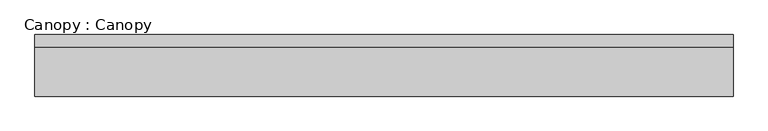
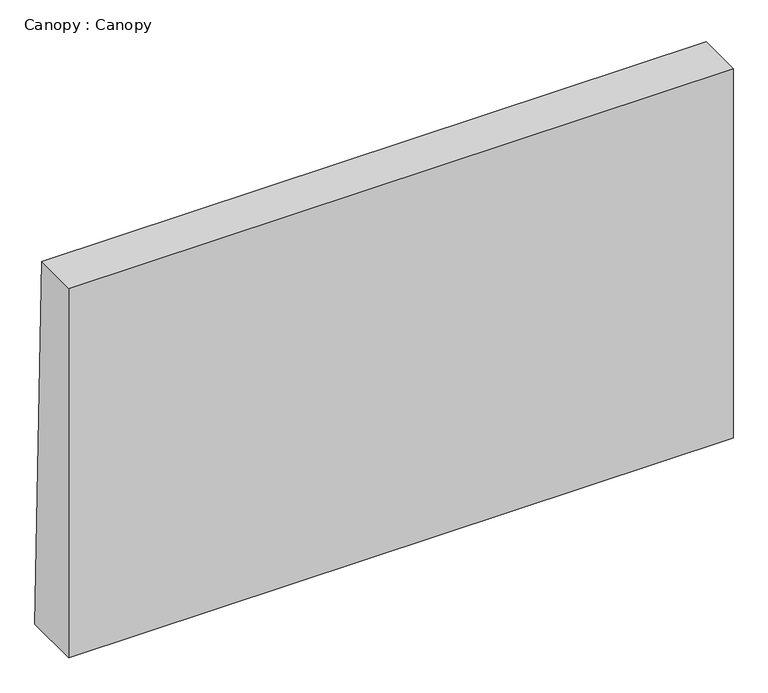
"""IFC4 building model written with IfcOpenShell, lengths in millimetres: proxy geometry, Canopy : Canopy."""

import ifcopenshell
import ifcopenshell.guid

model = None  # the IFC model being written
_history = None  # IfcOwnerHistory: only IFC2X3 demands one
_inside = {}  # id of a spatial element -> (the spatial element, [elements in it])
_under = {}  # id of a project, library or spatial element -> (it, [spatial elements below it])
_declared = {}  # id of a project -> (the project, [libraries it declares])
_typed = {}  # id of a type object -> (the type object, [elements of that type])
_made_of = {}  # id of a material, layer set ... -> (it, [elements and type objects made of it])


def new_model(schema):
    """Start an empty IFC model of exactly this schema.

    Asked for "IFC4X3", IfcOpenShell would pick the latest addendum, in which some entities
    have other attributes; the version numbers below select the first issue.
    IFC2X3 requires an IfcOwnerHistory on every rooted entity: one is made here for all.
    """
    global model, _history
    if schema == "IFC4X3":
        model = ifcopenshell.file(schema_version=(4, 3, 0, 0))
    else:
        model = ifcopenshell.file(schema=schema)
    _inside.clear()
    _under.clear()
    _declared.clear()
    _typed.clear()
    _made_of.clear()
    _history = None
    if model.schema == "IFC2X3":
        org = make("IfcOrganization", Name="unknown")
        user = make(
            "IfcPersonAndOrganization",
            ThePerson=make("IfcPerson", FamilyName="unknown"),
            TheOrganization=org,
        )
        app = make(
            "IfcApplication",
            ApplicationDeveloper=org,
            Version="unknown",
            ApplicationFullName="unknown",
            ApplicationIdentifier="unknown",
        )
        _history = make(
            "IfcOwnerHistory",
            OwningUser=user,
            OwningApplication=app,
            ChangeAction="ADDED",
            CreationDate=0,
        )
    return model


def make(cls, **values):
    """One entity of the class cls with the attributes given. An attribute that is None is left unset."""
    return model.create_entity(
        cls, **{name: value for name, value in values.items() if value is not None}
    )


def rooted(cls, **values):
    """An entity with a GlobalId (a new one), such as an element, a storey or a relation."""
    return make(cls, GlobalId=ifcopenshell.guid.new(), OwnerHistory=_history, **values)


def si_unit(unit_type, name, prefix=None):
    """IfcSIUnit, for example si_unit("LENGTHUNIT", "METRE", prefix="MILLI")."""
    return make("IfcSIUnit", UnitType=unit_type, Prefix=prefix, Name=name)


def assignment(units):
    """IfcUnitAssignment: the units of a project."""
    return None if units is None else make("IfcUnitAssignment", Units=units)


def point(xyz):
    """IfcCartesianPoint."""
    return None if xyz is None else make("IfcCartesianPoint", Coordinates=xyz)


def direction(xyz):
    """IfcDirection."""
    return None if xyz is None else make("IfcDirection", DirectionRatios=xyz)


def frame(location, z_axis=None, x_axis=None):
    """IfcAxis2Placement3D, a coordinate frame: its origin and axes. An axis left out is left unset."""
    return make(
        "IfcAxis2Placement3D",
        Location=point(location),
        Axis=direction(z_axis),
        RefDirection=direction(x_axis),
    )


def origin():
    """The frame at (0, 0, 0) with its axes left unset."""
    return frame((0.0, 0.0, 0.0))


def place(relative_to, where):
    """IfcLocalPlacement: puts the frame where relative to a parent placement (None: the world)."""
    return make(
        "IfcLocalPlacement", PlacementRelTo=relative_to, RelativePlacement=where
    )


def context(
    kind, dimensions, precision=None, world=None, true_north=None, identifier=None
):
    """IfcGeometricRepresentationContext, for example the 3D "Model" context."""
    return make(
        "IfcGeometricRepresentationContext",
        ContextIdentifier=identifier,
        ContextType=kind,
        CoordinateSpaceDimension=dimensions,
        Precision=precision,
        WorldCoordinateSystem=world,
        TrueNorth=true_north,
    )


def project(units=None, contexts=None):
    """IfcProject with its units and contexts."""
    return rooted(
        "IfcProject",
        Name="project",
        RepresentationContexts=contexts,
        UnitsInContext=assignment(units),
    )


def spatial(cls, under=None, at=None, **own):
    """A site, building, storey or space (cls), placed at a placement, below another one or the project."""
    s = rooted(cls, ObjectPlacement=at, **own)
    if under is not None:
        _under.setdefault(under.id(), (under, []))[1].append(s)
    return s


def polyline(points):
    """IfcPolyline through the points."""
    return make("IfcPolyline", Points=[point(p) for p in points])


def outline(outer, holes=None, kind="AREA"):
    """IfcArbitraryClosedProfileDef: a profile drawn as a closed curve; with holes, ...WithVoids."""
    if holes is None:
        return make("IfcArbitraryClosedProfileDef", ProfileType=kind, OuterCurve=outer)
    return make(
        "IfcArbitraryProfileDefWithVoids",
        ProfileType=kind,
        OuterCurve=outer,
        InnerCurves=holes,
    )


def extrude(swept, where, along, depth):
    """IfcExtrudedAreaSolid: the profile swept, set in the frame where, extruded along a direction by depth."""
    return make(
        "IfcExtrudedAreaSolid",
        SweptArea=swept,
        Position=where,
        ExtrudedDirection=direction(along),
        Depth=depth,
    )


def shape(context_of_items, identifier, shape_type, items):
    """IfcShapeRepresentation: the items that make up one representation, for example the "Body"."""
    return make(
        "IfcShapeRepresentation",
        ContextOfItems=context_of_items,
        RepresentationIdentifier=identifier,
        RepresentationType=shape_type,
        Items=items,
    )


def source(mapping_origin, context_of_items, identifier, shape_type, items):
    """IfcRepresentationMap: a shape defined once, which mapped items show again and again."""
    return make(
        "IfcRepresentationMap",
        MappingOrigin=mapping_origin,
        MappedRepresentation=shape(context_of_items, identifier, shape_type, items),
    )


def transform(
    local_origin,
    x_axis=None,
    y_axis=None,
    z_axis=None,
    scale=None,
    scale2=None,
    scale3=None,
    uniform=True,
):
    """IfcCartesianTransformationOperator3D, or its non-uniform kind. x_axis, y_axis, z_axis: its Axis1, 2, 3."""
    if uniform:
        return make(
            "IfcCartesianTransformationOperator3D",
            Axis1=direction(x_axis),
            Axis2=direction(y_axis),
            LocalOrigin=point(local_origin),
            Scale=scale,
            Axis3=direction(z_axis),
        )
    return make(
        "IfcCartesianTransformationOperator3DnonUniform",
        Axis1=direction(x_axis),
        Axis2=direction(y_axis),
        LocalOrigin=point(local_origin),
        Scale=scale,
        Axis3=direction(z_axis),
        Scale2=scale2,
        Scale3=scale3,
    )


def mapped(mapping_source, mapping_target):
    """IfcMappedItem: shows the shape of a source again, moved by a transform."""
    return make(
        "IfcMappedItem", MappingSource=mapping_source, MappingTarget=mapping_target
    )


def made_of(thing, what):
    """Note that an element or type object is made of a material, layer set ...; save() writes the relation."""
    if what is not None:
        _made_of.setdefault(what.id(), (what, []))[1].append(thing)
    return thing


def element(
    cls,
    number,
    at=None,
    inside=None,
    cuts=None,
    type_object=None,
    material=None,
    context=None,
    identifier="Body",
    shape_type=None,
    held_by="IfcProductDefinitionShape",
    body=None,
    shapes=None,
    **own,
):
    """One element of the class cls, such as IfcWall. Its Tag is "e" and its number.

    at: its placement. inside: the storey or other place that contains it. cuts: it is an
    opening in that element (IfcRelVoidsElement). A single representation is given by context,
    identifier, shape_type and body (its items); several are given by shapes. held_by: the class
    of the entity that holds the representations. save() writes the other relations.
    """
    e = rooted(cls, Tag="e%d" % number, ObjectPlacement=at, **own)
    if body is not None:
        shapes = [shape(context, identifier, shape_type, body)]
    if shapes is not None:
        e.Representation = make(held_by, Representations=shapes)
    if inside is not None:
        _inside.setdefault(inside.id(), (inside, []))[1].append(e)
    if cuts is not None:
        rooted(
            "IfcRelVoidsElement", RelatingBuildingElement=cuts, RelatedOpeningElement=e
        )
    if type_object is not None:
        _typed.setdefault(type_object.id(), (type_object, []))[1].append(e)
    return made_of(e, material)


def aggregate(whole, parts):
    """IfcRelAggregates: a whole, such as a stair, and the parts it consists of."""
    return rooted("IfcRelAggregates", RelatingObject=whole, RelatedObjects=parts)


def save(model, path):
    """Write the relations noted so far, then the file.

    IfcRelAggregates (storeys below a building ...), IfcRelContainedInSpatialStructure (elements
    in a storey), IfcRelDefinesByType, IfcRelAssociatesMaterial and IfcRelDeclares: one each for
    every whole, place, type object, material and project.
    """
    for whole, parts in _under.values():
        aggregate(whole, parts)
    for where, things in _inside.values():
        rooted(
            "IfcRelContainedInSpatialStructure",
            RelatedElements=things,
            RelatingStructure=where,
        )
    for kind, things in _typed.values():
        rooted("IfcRelDefinesByType", RelatedObjects=things, RelatingType=kind)
    for what, things in _made_of.values():
        rooted("IfcRelAssociatesMaterial", RelatedObjects=things, RelatingMaterial=what)
    for by, libraries in _declared.values():
        rooted("IfcRelDeclares", RelatingContext=by, RelatedDefinitions=libraries)
    model.write(path)


def canopy_canopy_239b8731(model_context):
    return source(origin(), model_context, "Body", "SweptSolid", [
        extrude(outline(polyline([(150.0, 0.0), (0.0, 0.0), (0.0, 1000.0), (120.0, 1000.0), (150.0, 0.0)])), frame((-850.0, 0.0, 0.0), z_axis=(1.0, 0.0, 0.0), x_axis=(0.0, 1.0, 0.0)), (0.0, 0.0, 1.0), 1700.0),
    ])


if __name__ == "__main__":
    model = new_model("IFC4")
    model_context = context("Model", 3, world=origin())
    ifc_project = project(units=[si_unit("LENGTHUNIT", "METRE", prefix="MILLI")], contexts=[model_context])
    site = spatial("IfcSite", under=ifc_project)
    building = spatial("IfcBuilding", under=site)
    placement = place(None, origin())
    canopy_canopy_shape = canopy_canopy_239b8731(model_context)
    element("IfcBuildingElementProxy", 1, Name="Canopy : Canopy", ObjectType="Canopy : Canopy", at=placement, inside=building, context=model_context, shape_type="MappedRepresentation", body=[
        mapped(canopy_canopy_shape, transform((0.0, 0.0, 0.0), x_axis=(1.0, 0.0, 0.0), y_axis=(0.0, 1.0, 0.0), z_axis=(0.0, 0.0, 1.0))),
    ])
    save(model, "model.ifc")

# Revit data of these elements
# Type "Canopy : Canopy"
#   Type Comments = "CV-AG"
#   H_Rebar Ratio = 0.1
#   Canopy Width [instance default] = 1700 mm
#   Canopy Length [instance default] = 1000 mm
#   Canopy L.P = 120 mm
#   Canopy H.P = 150 mm
#   구조재료 = Concrete_f'c=28MPa(Cylender)
#   Default Elevation = 0
# Element 1 (IfcBuildingElementProxy, "Canopy : Canopy")
#   Materials on its faces: "Concrete_f'c=28MPa(Cylender)"
# Materials
#   "Concrete_f'c=28MPa(Cylender)": class "Concrete", colour RGB 176 176 176, transparency 0, Description = "Reinf. Conc.", Cost = 0, Image = Concrete.Cast-In-Place.Flat.Polished.Grey.jpg
